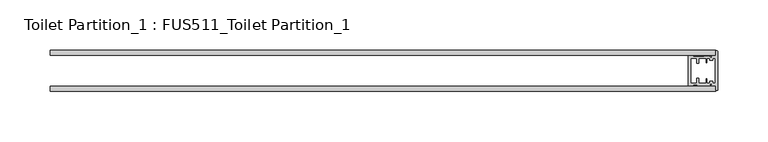
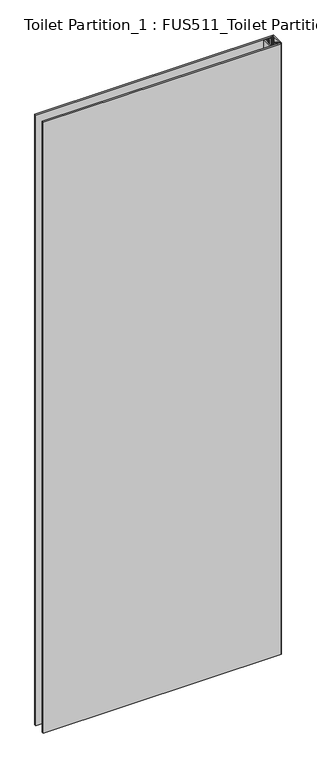
"""IFC4 building model written with IfcOpenShell, lengths in millimetres: furniture geometry, Toilet Partition_1 : FUS511_Toilet Partition_1."""

from ifc_helpers import new_model, si_unit, point, frame, frame_2d, origin, place, context, project, spatial, polyline, circle_curve, trimmed, segment, composite_curve, outline, extrude, source, transform, mapped, element, save


def toilet_partition_1_fus511_toilet_partition_1_37ce349d(model_context):
    return source(origin(), model_context, "Body", "SweptSolid", [
        extrude(outline(composite_curve([segment(polyline([(292.1234192, 489.5206414), (297.0588506, 489.5206414), (297.0588506, 488.5335551), (301.0071958, 488.5335551), (314.5796324, 489.5206414)]), True, "CONTINUOUS"), segment(trimmed(circle_curve(frame_2d((314.8264039, 488.5648992)), 0.9870863), [point((314.5796324, 489.5206414))], [point((315.0731755, 489.5206414))], True, "CARTESIAN"), True, "CONTINUOUS"), segment(polyline([(315.0731755, 489.5206414), (319.7618354, 489.5206414), (319.7618354, 494.4560729), (320.7489217, 494.4560729)]), True, "CONTINUOUS"), segment(trimmed(circle_curve(frame_2d((320.7489217, 493.4689866)), 0.9870863), [point((320.7489217, 494.4560729))], [point((321.736008, 493.4689866))], False, "CARTESIAN"), True, "CONTINUOUS"), segment(polyline([(321.736008, 493.4689866), (321.736008, 455.9597074)]), True, "CONTINUOUS"), segment(trimmed(circle_curve(frame_2d((320.7489217, 455.9597074)), 0.9870863), [point((321.736008, 455.9597074))], [point((320.7489217, 454.9726211))], False, "CARTESIAN"), True, "CONTINUOUS"), segment(polyline([(320.7489217, 454.9726211), (319.7618354, 454.9726211), (319.7618354, 459.9080525), (315.0731755, 459.9080525)]), True, "CONTINUOUS"), segment(trimmed(circle_curve(frame_2d((314.8264039, 460.8637947)), 0.9870863), [point((315.0731755, 459.9080525))], [point((314.5796324, 459.9080525))], True, "CARTESIAN"), True, "CONTINUOUS"), segment(polyline([(314.5796324, 459.9080525), (301.0071958, 459.9080525), (301.0071958, 460.8951388), (297.0588506, 460.8951388), (297.0588506, 459.9080525), (292.1234192, 459.9080525), (292.1234192, 489.5206414)]), True, "CONTINUOUS")], self_intersect=False), holes=[polyline([(295.084678, 486.5593825), (295.084678, 462.8693114), (300.0201095, 462.8693114), (300.0201095, 467.8047429), (302.9813684, 467.8047429), (302.9813684, 462.8693114), (309.8909725, 462.8693114), (309.8909725, 467.3111998), (311.3716019, 467.3111998), (311.3716019, 462.8693114), (313.0990029, 462.8693114), (313.0990029, 464.843484), (317.0473481, 464.843484), (317.0473481, 462.8693114), (318.7747491, 462.8693114), (318.7747491, 486.5593825), (317.0473481, 486.5593825), (317.0473481, 484.5852099), (313.0990029, 484.5852099), (313.0990029, 486.5593825), (311.3716019, 486.5593825), (311.3716019, 482.1174942), (309.8909725, 482.1174942), (309.8909725, 486.5593825), (302.9813684, 486.5593825), (302.9813684, 481.623951), (300.0201095, 481.623951), (300.0201095, 486.5593825), (295.084678, 486.5593825)])]), frame((0.0, 0.0, 100.0), z_axis=(0.0, 0.0, 1.0), x_axis=(1.0, 0.0, 0.0)), (0.0, 0.0, 1.0), 1800.0),
        extrude(outline(polyline([(-344.2381646, 454.214347), (-344.2381646, 459.214347), (319.7618354, 459.214347), (319.7618354, 454.214347), (-344.2381646, 454.214347)])), frame((0.0, 0.0, 100.0), z_axis=(0.0, 0.0, 1.0), x_axis=(1.0, 0.0, 0.0)), (0.0, 0.0, 1.0), 1800.0),
        extrude(outline(polyline([(-344.2381646, 490.214347), (-344.2381646, 495.214347), (319.7618354, 495.214347), (319.7618354, 490.214347), (-344.2381646, 490.214347)])), frame((0.0, 0.0, 100.0), z_axis=(0.0, 0.0, 1.0), x_axis=(1.0, 0.0, 0.0)), (0.0, 0.0, 1.0), 1800.0),
    ])


if __name__ == "__main__":
    model = new_model("IFC4")
    model_context = context("Model", 3, world=origin())
    ifc_project = project(units=[si_unit("LENGTHUNIT", "METRE", prefix="MILLI")], contexts=[model_context])
    site = spatial("IfcSite", under=ifc_project)
    building = spatial("IfcBuilding", under=site)
    placement = place(None, origin())
    toilet_partition_1_fus511_toilet_partition_1_shape = toilet_partition_1_fus511_toilet_partition_1_37ce349d(model_context)
    element("IfcFurniture", 1, ObjectType="Toilet Partition_1 : FUS511_Toilet Partition_1", at=placement, inside=building, context=model_context, shape_type="MappedRepresentation", body=[
        mapped(toilet_partition_1_fus511_toilet_partition_1_shape, transform((0.0, 0.0, 0.0), x_axis=(1.0, 0.0, 0.0), y_axis=(0.0, 1.0, 0.0), z_axis=(0.0, 0.0, 1.0))),
    ])
    save(model, "model.ifc")

# Revit data of these elements
# Type "Toilet Partition_1 : FUS511_Toilet Partition_1"
#   Created by = "Utku Can Kocadağ"
#   Controlled by = "Sefer Özdoğan"
#   Approved by = "Aydın Altınova"
#   Cubicle_Height = 1800 mm
#   Bot_Gap = 100 mm
#   Default Elevation = 0
# Element 1 (IfcFurniture, "Toilet Partition_1 : FUS511_Toilet Partition_1")
#   Materials on its faces: "Aln_Aluminum_02"
# Materials
#   "Aln_Aluminum_02": class "Generic", colour RGB 120 120 120, transparency 0, Cost = 0
